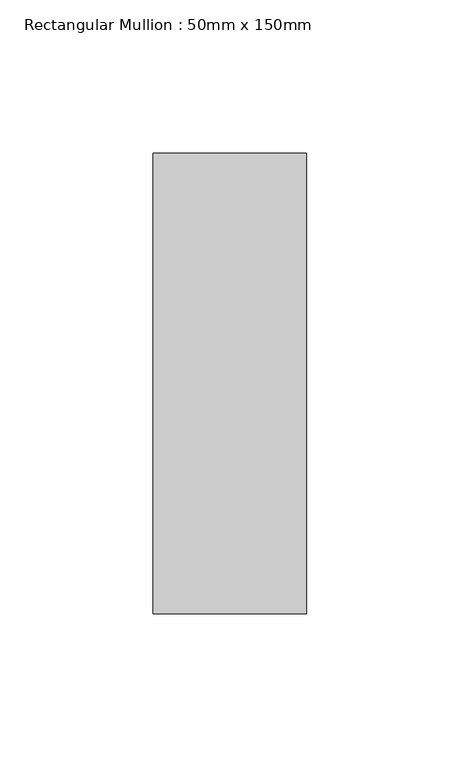
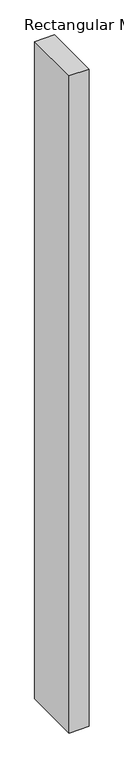
"""IFC4 building model written with IfcOpenShell, lengths in millimetres: member geometry, Rectangular Mullion : 50mm x 150mm."""

from ifc_helpers import new_model, si_unit, frame, origin, place, context, project, spatial, polyline, outline, extrude, source, transform, mapped, element, save


def rectangular_mullion_50mm_x_150mm_f862f7d9(model_context):
    return source(origin(), model_context, "Body", "SweptSolid", [
        extrude(outline(polyline([(25.0, 75.0), (25.0, -75.0), (-25.0, -75.0), (-25.0, 75.0), (25.0, 75.0)])), frame((0.0, 0.0, -1740.2939092), z_axis=(0.0, 0.0, 1.0), x_axis=(1.0, 0.0, 0.0)), (0.0, 0.0, 1.0), 1740.2939092),
    ])


if __name__ == "__main__":
    model = new_model("IFC4")
    model_context = context("Model", 3, world=origin())
    ifc_project = project(units=[si_unit("LENGTHUNIT", "METRE", prefix="MILLI")], contexts=[model_context])
    site = spatial("IfcSite", under=ifc_project)
    building = spatial("IfcBuilding", under=site)
    placement = place(None, origin())
    rectangular_mullion_50mm_x_150mm_shape = rectangular_mullion_50mm_x_150mm_f862f7d9(model_context)
    element("IfcMember", 1, ObjectType="Rectangular Mullion : 50mm x 150mm", at=placement, inside=building, context=model_context, shape_type="MappedRepresentation", body=[
        mapped(rectangular_mullion_50mm_x_150mm_shape, transform((0.0, 0.0, 0.0), x_axis=(1.0, 0.0, 0.0), y_axis=(0.0, 1.0, 0.0), z_axis=(0.0, 0.0, 1.0))),
    ])
    save(model, "model.ifc")

# Revit data of these elements
# Type "Rectangular Mullion : 50mm x 150mm"
#   built-in parameter 1007304 = 0.492126 (stored number, unit not read)
#   built-in parameter 1007301 = 0.082021 (stored number, unit not read)
#   built-in parameter 1007300 = 0.082021 (stored number, unit not read)
# Element 1 (IfcMember, "Rectangular Mullion : 50mm x 150mm")
#   Materials on its faces: "Aluminum"
# Materials
#   "Aluminum": class "Metal", colour RGB 244 244 244, transparency 0, Description = "Aluminum 6061", Cost = 0
